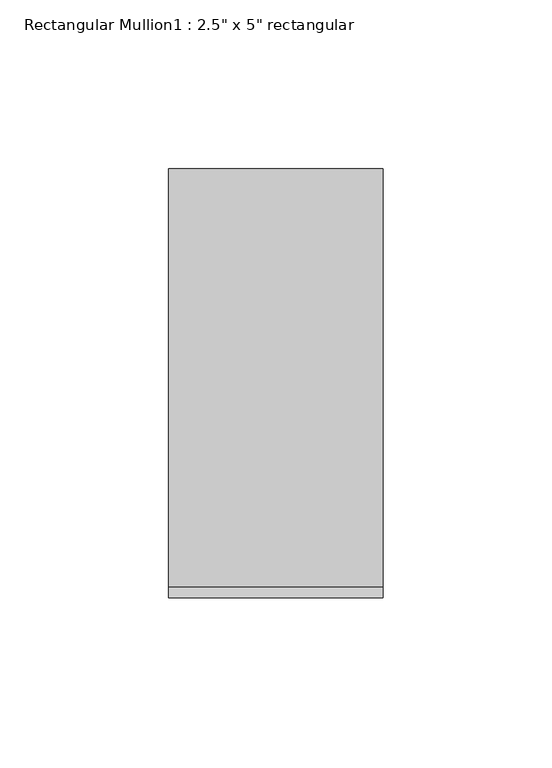
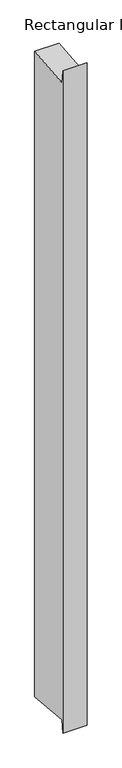
"""IFC4 building model written with IfcOpenShell, lengths in millimetres: member geometry."""

from ifc_helpers import new_model, si_unit, frame, origin, place, context, project, spatial, polyline, outline, extrude, source, transform, mapped, element, save


def member_b9454cfc(model_context):
    return source(origin(), model_context, "Body", "SweptSolid", [
        extrude(outline(polyline([(-63.5, 28.7582862), (-60.2336356, -5.8295375), (63.5, 5.8554746), (63.5, -1771.1554746), (-60.2336356, -1759.4704625), (-63.5, -1794.0582862), (-63.5, 28.7582862)])), frame((-63.5, 0.0, 0.0), z_axis=(1.0, 0.0, 0.0), x_axis=(0.0, 1.0, 0.0)), (0.0, 0.0, 1.0), 63.5),
    ])


if __name__ == "__main__":
    model = new_model("IFC4")
    model_context = context("Model", 3, world=origin())
    ifc_project = project(units=[si_unit("LENGTHUNIT", "METRE", prefix="MILLI")], contexts=[model_context])
    site = spatial("IfcSite", under=ifc_project)
    building = spatial("IfcBuilding", under=site)
    placement = place(None, origin())
    member_shape = member_b9454cfc(model_context)
    element("IfcMember", 1, ObjectType="Rectangular Mullion1 : 2.5\" x 5\" rectangular", at=placement, inside=building, context=model_context, shape_type="MappedRepresentation", body=[
        mapped(member_shape, transform((0.0, 0.0, 0.0), x_axis=(1.0, 0.0, 0.0), y_axis=(0.0, 1.0, 0.0), z_axis=(0.0, 0.0, 1.0))),
    ])
    save(model, "model.ifc")

# Revit data of these elements
# Type "Rectangular Mullion1 : 2.5\" x 5\" rectangular"
#   built-in parameter 1007304 = 0.416667 (stored number, unit not read)
#   built-in parameter 1007301 = 0.104167 (stored number, unit not read)
#   built-in parameter 1007300 = 0.104167 (stored number, unit not read)
# Element 1 (IfcMember, "Rectangular Mullion1 : 2.5\" x 5\" rectangular")
#   Materials on its faces: "support-frame"
# Materials
#   "support-frame": class "Unassigned", colour RGB 233 233 233, transparency 0, Cost = 0
